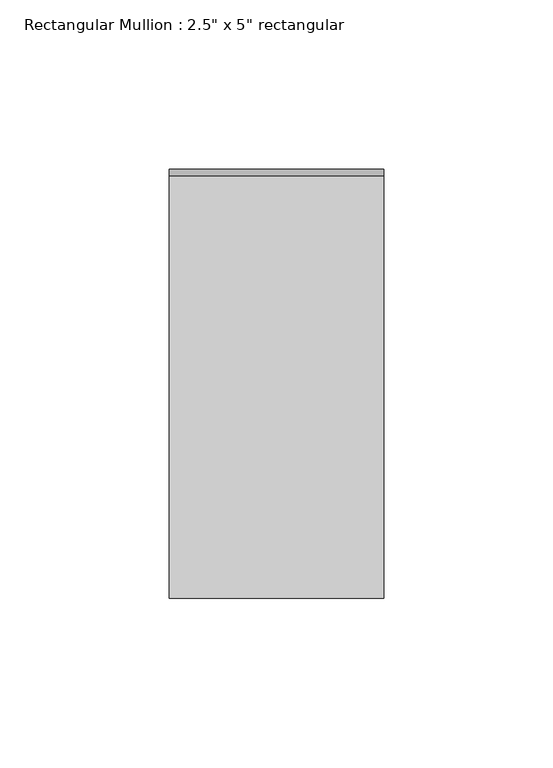
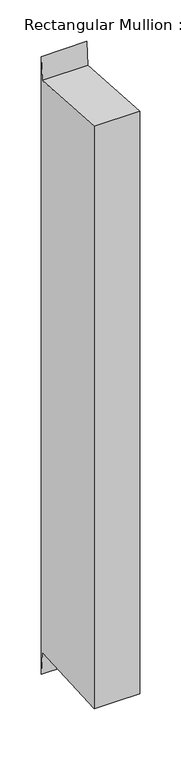
"""IFC4 building model written with IfcOpenShell, lengths in millimetres: member geometry."""

from ifc_helpers import new_model, si_unit, origin, place, context, project, spatial, faceted_brep, source, transform, mapped, element, save


def member_6ad7a984(model_context):
    return source(origin(), model_context, "Body", "Brep", [
        faceted_brep([(-31.75, 63.5, 29.7846233), (31.75, 63.5, 29.7846233), (31.75, 63.5, -880.6846233), (0.0, 63.5, -880.6846233), (-31.75, 63.5, -880.6846233), (-31.75, -63.5, 3.8736342), (-31.75, 61.4149606, -3.8662198), (-31.75, 61.4149606, -847.0337802), (-31.75, -63.5, -854.7736342), (31.75, -63.5, 3.8736342), (0.0, -63.5, -854.7736342), (31.75, -63.5, -854.7736342), (31.75, 61.4149606, -3.8662198), (31.75, 61.4149606, -847.0337802), (0.0, 61.4149606, -847.0337802)], [[[0, 1, 2, 3, 4]], [[5, 6, 0, 4, 7, 8]], [[9, 5, 8, 10, 11]], [[1, 12, 9, 11, 13, 2]], [[1, 0, 6, 12]], [[6, 5, 9, 12]], [[2, 13, 14, 3]], [[13, 11, 10, 14]], [[10, 8, 7, 14]], [[7, 4, 3, 14]]]),
    ])


if __name__ == "__main__":
    model = new_model("IFC4")
    model_context = context("Model", 3, world=origin())
    ifc_project = project(units=[si_unit("LENGTHUNIT", "METRE", prefix="MILLI")], contexts=[model_context])
    site = spatial("IfcSite", under=ifc_project)
    building = spatial("IfcBuilding", under=site)
    placement = place(None, origin())
    member_shape = member_6ad7a984(model_context)
    element("IfcMember", 1, ObjectType="Rectangular Mullion : 2.5\" x 5\" rectangular", at=placement, inside=building, context=model_context, shape_type="MappedRepresentation", body=[
        mapped(member_shape, transform((0.0, 0.0, 0.0), x_axis=(1.0, 0.0, 0.0), y_axis=(0.0, 1.0, 0.0), z_axis=(0.0, 0.0, 1.0))),
    ])
    save(model, "model.ifc")

# Revit data of these elements
# Type "Rectangular Mullion : 2.5\" x 5\" rectangular"
#   built-in parameter 1007304 = 0.416667 (stored number, unit not read)
#   built-in parameter 1007301 = 0.104167 (stored number, unit not read)
#   built-in parameter 1007300 = 0.104167 (stored number, unit not read)
# Element 1 (IfcMember, "Rectangular Mullion : 2.5\" x 5\" rectangular")
#   Materials on its faces: "Metal - Aluminum"
# Materials
#   "Metal - Aluminum": class "Metal", colour RGB 247 247 247, transparency 0, Cost = 0
